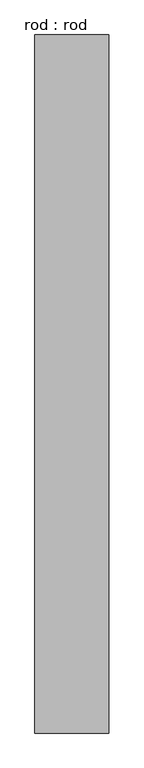
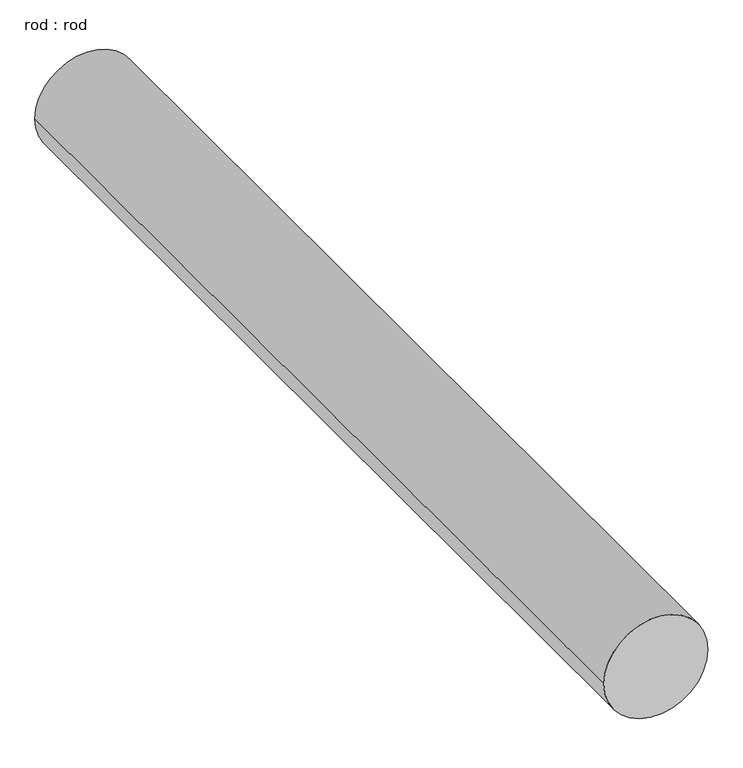
"""IFC4 building model written with IfcOpenShell, lengths in millimetres: proxy geometry, rod : rod."""

from ifc_helpers import new_model, si_unit, point, frame, frame_2d, origin, place, context, project, spatial, circle_curve, trimmed, segment, composite_curve, outline, extrude, source, transform, mapped, element, save


def rod_rod_cb86c36d(model_context):
    return source(origin(), model_context, "Body", "SweptSolid", [
        extrude(outline(composite_curve([segment(trimmed(circle_curve(frame_2d((0.0108462, 0.0)), 200.0), [point((0.0108462, 200.0))], [point((0.0108462, -200.0))], False, "CARTESIAN"), True, "CONTINUOUS"), segment(trimmed(circle_curve(frame_2d((0.0108462, 0.0)), 200.0), [point((0.0108462, -200.0))], [point((0.0108462, 200.0))], False, "CARTESIAN"), True, "CONTINUOUS")], self_intersect=False)), frame((0.0, 2199.6678004, 0.0), z_axis=(0.0, 1.0, 0.0), x_axis=(0.0, 0.0, 1.0)), (0.0, 0.0, 1.0), 3786.1216299),
    ])


if __name__ == "__main__":
    model = new_model("IFC4")
    model_context = context("Model", 3, world=origin())
    ifc_project = project(units=[si_unit("LENGTHUNIT", "METRE", prefix="MILLI")], contexts=[model_context])
    site = spatial("IfcSite", under=ifc_project)
    building = spatial("IfcBuilding", under=site)
    placement = place(None, origin())
    rod_rod_shape = rod_rod_cb86c36d(model_context)
    element("IfcBuildingElementProxy", 1, Name="rod : rod", ObjectType="rod : rod", at=placement, inside=building, context=model_context, shape_type="MappedRepresentation", body=[
        mapped(rod_rod_shape, transform((0.0, 0.0, 0.0), x_axis=(1.0, 0.0, 0.0), y_axis=(0.0, 1.0, 0.0), z_axis=(0.0, 0.0, 1.0))),
    ])
    save(model, "model.ifc")

# Revit data of these elements
# Type "rod : rod"
#   Default Elevation = 0
